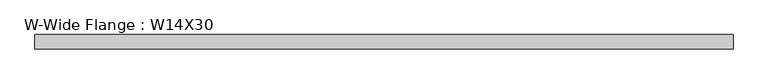
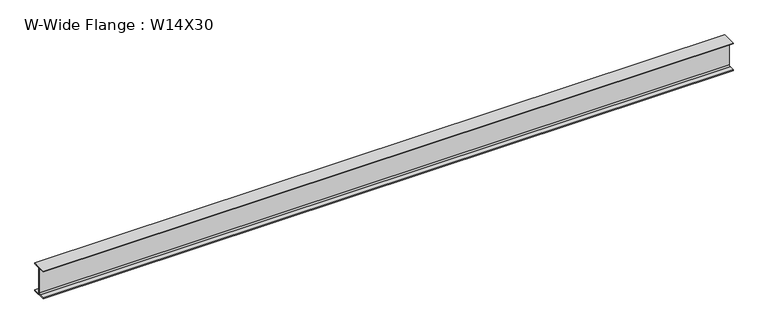
"""IFC4 building model written with IfcOpenShell, lengths in millimetres: beam geometry, W-Wide Flange : W14X30."""

from ifc_helpers import new_model, si_unit, point, frame, frame_2d, origin, place, context, project, spatial, polyline, circle_curve, trimmed, segment, composite_curve, outline, extrude, source, transform, mapped, element, save


def w_wide_flange_w14x30_a3fd6266(model_context):
    return source(origin(), model_context, "Body", "SweptSolid", [
        extrude(outline(composite_curve([segment(polyline([(85.4769531, -165.9433594), (85.4769531, -175.7660156), (-85.4769531, -175.7660156), (-85.4769531, -165.9433594), (-22.1753906, -165.9433594)]), True, "CONTINUOUS"), segment(trimmed(circle_curve(frame_2d((-22.1753906, -147.1910156)), 18.7523438), [point((-22.1753906, -165.9433594))], [point((-3.4230469, -147.1910156))], True, "CARTESIAN"), True, "CONTINUOUS"), segment(polyline([(-3.4230469, -147.1910156), (-3.4230469, 147.1910156)]), True, "CONTINUOUS"), segment(trimmed(circle_curve(frame_2d((-22.1753906, 147.1910156)), 18.7523438), [point((-3.4230469, 147.1910156))], [point((-22.1753906, 165.9433594))], True, "CARTESIAN"), True, "CONTINUOUS"), segment(polyline([(-22.1753906, 165.9433594), (-85.4769531, 165.9433594), (-85.4769531, 175.7660156), (85.4769531, 175.7660156), (85.4769531, 165.9433594), (22.1753906, 165.9433594)]), True, "CONTINUOUS"), segment(trimmed(circle_curve(frame_2d((22.1753906, 147.1910156)), 18.7523438), [point((22.1753906, 165.9433594))], [point((3.4230469, 147.1910156))], True, "CARTESIAN"), True, "CONTINUOUS"), segment(polyline([(3.4230469, 147.1910156), (3.4230469, -147.1910156)]), True, "CONTINUOUS"), segment(trimmed(circle_curve(frame_2d((22.1753906, -147.1910156)), 18.7523438), [point((3.4230469, -147.1910156))], [point((22.1753906, -165.9433594))], True, "CARTESIAN"), True, "CONTINUOUS"), segment(polyline([(22.1753906, -165.9433594), (85.4769531, -165.9433594)]), True, "CONTINUOUS")], self_intersect=False)), frame((-4102.4594962, 0.0, 0.0), z_axis=(1.0, 0.0, 0.0), x_axis=(0.0, 1.0, 0.0)), (0.0, 0.0, 1.0), 8300.4229925),
    ])


if __name__ == "__main__":
    model = new_model("IFC4")
    model_context = context("Model", 3, world=origin())
    ifc_project = project(units=[si_unit("LENGTHUNIT", "METRE", prefix="MILLI")], contexts=[model_context])
    site = spatial("IfcSite", under=ifc_project)
    building = spatial("IfcBuilding", under=site)
    placement = place(None, origin())
    w_wide_flange_w14x30_shape = w_wide_flange_w14x30_a3fd6266(model_context)
    element("IfcBeam", 1, ObjectType="W-Wide Flange : W14X30", at=placement, inside=building, context=model_context, shape_type="MappedRepresentation", body=[
        mapped(w_wide_flange_w14x30_shape, transform((0.0, 0.0, 0.0), x_axis=(1.0, 0.0, 0.0), y_axis=(0.0, 1.0, 0.0), z_axis=(0.0, 0.0, 1.0))),
    ])
    save(model, "model.ifc")

# Revit data of these elements
# Type "W-Wide Flange : W14X30"
#   Assembly Code = "B10"
#   W = 30
#   Length [instance default] = 1524 mm
#   bf = 170.954 mm
#   d = 351.532 mm
#   k = 28.575 mm
#   k2 = 18.752 mm
#   tf = 9.823 mm
#   tw = 6.846 mm
#   A = 0.00557418 m²
#   Structural Material [instance default] = Steel ASTM A992
# Element 1 (IfcBeam, "W-Wide Flange : W14X30")
#   Structural Material = Aluminum, Anodized Red
#   Materials on its faces: "Aluminum, Anodized Red"
# Materials
#   "Steel ASTM A992": class "Metal", colour RGB 128 0 0, transparency 0, Description = "Structural steel 50ksi", Cost = 0
#   "Aluminum, Anodized Red": class "Metal", colour RGB 120 120 120, transparency 0, Description = "Anodized aluminum, red", Cost = 0
